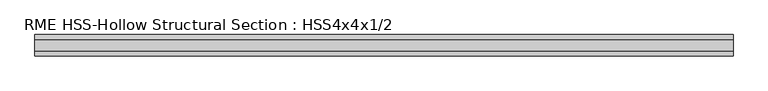
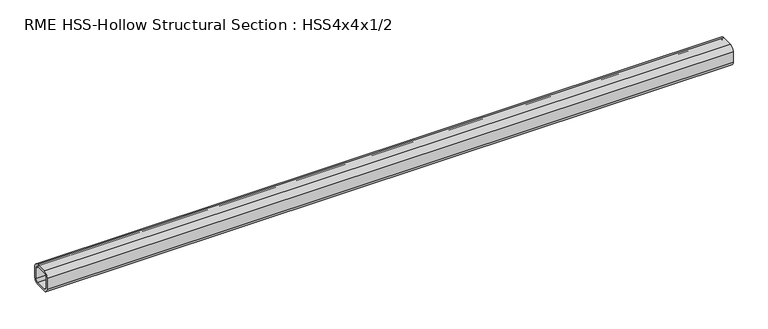
"""IFC4 building model written with IfcOpenShell, lengths in millimetres: member geometry, RME HSS-Hollow Structural Section : HSS4x4x1/2."""

from ifc_helpers import new_model, si_unit, point, frame, frame_2d, origin, place, context, project, spatial, polyline, circle_curve, trimmed, segment, composite_curve, outline, extrude, source, transform, mapped, element, save


def rme_hss_hollow_structural_section_hss4x4x1_2_02136324(model_context):
    return source(origin(), model_context, "Body", "SweptSolid", [
        extrude(outline(composite_curve([segment(polyline([(50.8, 27.178), (50.8, -27.178)]), True, "CONTINUOUS"), segment(trimmed(circle_curve(frame_2d((27.178, -27.178)), 23.622), [point((50.8, -27.178))], [point((27.178, -50.8))], False, "CARTESIAN"), True, "CONTINUOUS"), segment(polyline([(27.178, -50.8), (-27.178, -50.8)]), True, "CONTINUOUS"), segment(trimmed(circle_curve(frame_2d((-27.178, -27.178)), 23.622), [point((-27.178, -50.8))], [point((-50.8, -27.178))], False, "CARTESIAN"), True, "CONTINUOUS"), segment(polyline([(-50.8, -27.178), (-50.8, 27.178)]), True, "CONTINUOUS"), segment(trimmed(circle_curve(frame_2d((-27.178, 27.178)), 23.622), [point((-50.8, 27.178))], [point((-27.178, 50.8))], False, "CARTESIAN"), True, "CONTINUOUS"), segment(polyline([(-27.178, 50.8), (27.178, 50.8)]), True, "CONTINUOUS"), segment(trimmed(circle_curve(frame_2d((27.178, 27.178)), 23.622), [point((27.178, 50.8))], [point((50.8, 27.178))], False, "CARTESIAN"), True, "CONTINUOUS")], self_intersect=False), holes=[composite_curve([segment(trimmed(circle_curve(frame_2d((-27.178, 27.178)), 11.811), [point((-27.178, 38.989))], [point((-38.989, 27.178))], True, "CARTESIAN"), True, "CONTINUOUS"), segment(polyline([(-38.989, 27.178), (-38.989, -27.178)]), True, "CONTINUOUS"), segment(trimmed(circle_curve(frame_2d((-27.178, -27.178)), 11.811), [point((-38.989, -27.178))], [point((-27.178, -38.989))], True, "CARTESIAN"), True, "CONTINUOUS"), segment(polyline([(-27.178, -38.989), (27.178, -38.989)]), True, "CONTINUOUS"), segment(trimmed(circle_curve(frame_2d((27.178, -27.178)), 11.811), [point((27.178, -38.989))], [point((38.989, -27.178))], True, "CARTESIAN"), True, "CONTINUOUS"), segment(polyline([(38.989, -27.178), (38.989, 27.178)]), True, "CONTINUOUS"), segment(trimmed(circle_curve(frame_2d((27.178, 27.178)), 11.811), [point((38.989, 27.178))], [point((27.178, 38.989))], True, "CARTESIAN"), True, "CONTINUOUS"), segment(polyline([(27.178, 38.989), (-27.178, 38.989)]), True, "CONTINUOUS")], self_intersect=False)]), frame((-1745.7935577, 0.0, 0.0), z_axis=(1.0, 0.0, 0.0), x_axis=(0.0, 1.0, 0.0)), (0.0, 0.0, 1.0), 3298.7896683),
    ])


if __name__ == "__main__":
    model = new_model("IFC4")
    model_context = context("Model", 3, world=origin())
    ifc_project = project(units=[si_unit("LENGTHUNIT", "METRE", prefix="MILLI")], contexts=[model_context])
    site = spatial("IfcSite", under=ifc_project)
    building = spatial("IfcBuilding", under=site)
    placement = place(None, origin())
    rme_hss_hollow_structural_section_hss4x4x1_2_shape = rme_hss_hollow_structural_section_hss4x4x1_2_02136324(model_context)
    element("IfcMember", 1, ObjectType="RME HSS-Hollow Structural Section : HSS4x4x1/2", at=placement, inside=building, context=model_context, shape_type="MappedRepresentation", body=[
        mapped(rme_hss_hollow_structural_section_hss4x4x1_2_shape, transform((0.0, 0.0, 0.0), x_axis=(1.0, 0.0, 0.0), y_axis=(0.0, 1.0, 0.0), z_axis=(0.0, 0.0, 1.0))),
    ])
    save(model, "model.ifc")

# Revit data of these elements
# Type "RME HSS-Hollow Structural Section : HSS4x4x1/2"
#   Nominal Size = "HSS6x4"
#   Assembly Code = "B10"
#   Shape = "Square"
#   W = 21.5
#   Start Extension Calculation [instance default] = 10' - 0"
#   Start Extension [instance default] = -0' - 0 1/2"
#   End Extension Calculation [instance default] = 10' - 0"
#   End Extension [instance default] = -0' - 0 1/2"
#   Ht = 0' - 4"
#   Length [instance default] = 5' - 0"
#   b = 0' - 4"
#   kr = 0' - 0.93"
#   t = 0' - 0.465"
#   A = 0.0418056 SF
#   Structural Material [instance default] = Metal - Steel - ASTM A500 - Grade B - Rectangular and Square
# Element 1 (IfcMember, "RME HSS-Hollow Structural Section : HSS4x4x1/2")
#   Structural Material = Metal - Steel - ASTM A992
#   Materials on its faces: "Metal - Steel - ASTM A992"
# Materials
#   "Metal - Steel - ASTM A500 - Grade B - Rectangular and Square": class "Metal", colour RGB 255 128 0, transparency 0
#   "Metal - Steel - ASTM A992": class "Metal", colour RGB 255 128 0, transparency 0
